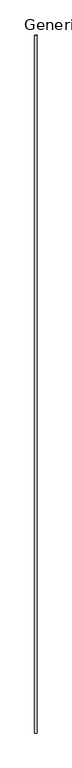
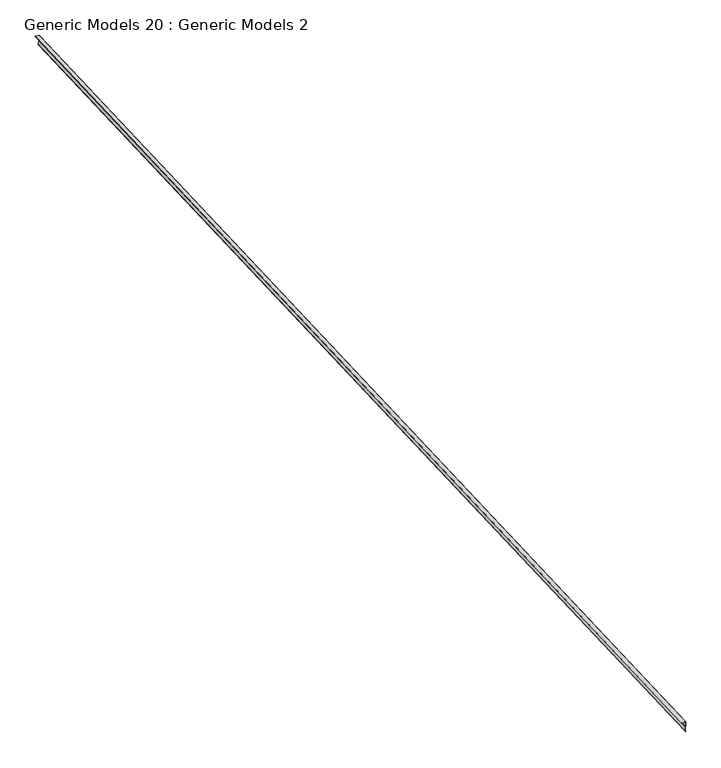
"""IFC4 building model written with IfcOpenShell, lengths in millimetres: proxy geometry, Generic Models 20 : Generic Models 2."""

from ifc_helpers import new_model, si_unit, frame, origin, place, context, project, spatial, polyline, outline, extrude, source, transform, mapped, element, save


def generic_models_20_generic_models_2_8eab422f(model_context):
    return source(origin(), model_context, "Body", "SweptSolid", [
        extrude(outline(polyline([(-13.3278111, -1e-07), (0.0, 0.0), (0.0, -1.5875001), (-14.9153111, -1.5875), (-14.9153112, 3.6817408), (2.820085, 3.6817409), (100.6729663, 101.5346222), (100.6729663, 116.8722084), (203.2763652, 219.4756072), (286.3437343, 136.4082381), (280.6506426, 130.7151464), (264.6713848, 146.6944042), (265.7939168, 147.8169362), (280.6506426, 132.9602104), (284.0986703, 136.4082381), (203.2763652, 217.2305432), (102.2604663, 116.2146444), (102.2604664, 100.8770582), (3.477649, 2.0942409), (-13.3278112, 2.0942408), (-13.3278111, -1e-07)])), frame((667610.426049, -569973.3361981, 8555.3813571), z_axis=(0.0, 0.9991330730923522, 0.04163054471217685), x_axis=(-0.7071067811890491, -0.029437240470365878, 0.7064937712888574)), (0.0, 0.0, 1.0), 33406.7702703),
    ])


if __name__ == "__main__":
    model = new_model("IFC4")
    model_context = context("Model", 3, world=origin())
    ifc_project = project(units=[si_unit("LENGTHUNIT", "METRE", prefix="MILLI")], contexts=[model_context])
    site = spatial("IfcSite", under=ifc_project)
    building = spatial("IfcBuilding", under=site)
    placement = place(None, origin())
    generic_models_20_generic_models_2_shape = generic_models_20_generic_models_2_8eab422f(model_context)
    element("IfcBuildingElementProxy", 1, Name="Generic Models 20 : Generic Models 2", ObjectType="Generic Models 20 : Generic Models 2", at=placement, inside=building, context=model_context, shape_type="MappedRepresentation", body=[
        mapped(generic_models_20_generic_models_2_shape, transform((0.0, 0.0, 0.0), x_axis=(1.0, 0.0, 0.0), y_axis=(0.0, 1.0, 0.0), z_axis=(0.0, 0.0, 1.0))),
    ])
    save(model, "model.ifc")

# Revit data of these elements
# Element 1 (IfcBuildingElementProxy, "Generic Models 20 : Generic Models 2")
#   Materials on its faces: "RAKE TRIM"
# Materials
#   "RAKE TRIM": class "Unassigned", colour RGB 210 209 208, transparency 0, Cost = 0
